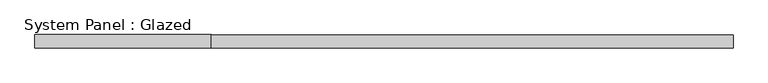
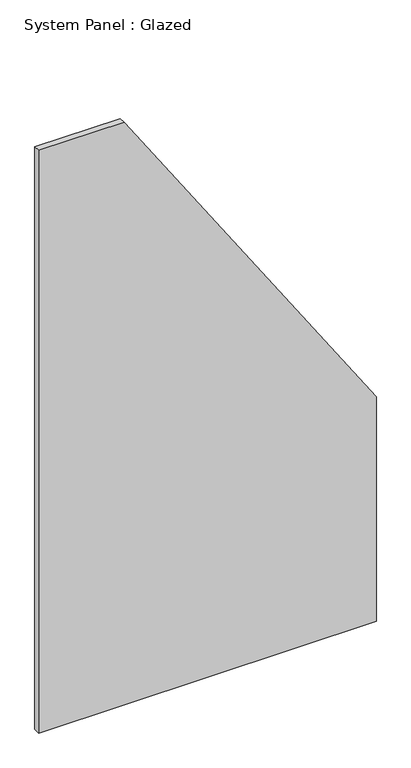
"""IFC4 building model written with IfcOpenShell, lengths in millimetres: plate geometry, System Panel : Glazed."""

from ifc_helpers import new_model, si_unit, frame, origin, place, context, project, spatial, polyline, outline, extrude, source, transform, mapped, element, save


def system_panel_glazed_e9d80b72(model_context):
    return source(origin(), model_context, "Body", "SweptSolid", [
        extrude(outline(polyline([(0.0, -658.3333333), (0.0, 658.3333333), (924.6254194, 658.3333333), (2400.0, -325.3849432), (2400.0, -658.3333333), (0.0, -658.3333333)])), frame((0.0, 24.5, 0.0), z_axis=(0.0, 1.0, 0.0), x_axis=(0.0, 0.0, 1.0)), (0.0, 0.0, 1.0), 25.0),
    ])


if __name__ == "__main__":
    model = new_model("IFC4")
    model_context = context("Model", 3, world=origin())
    ifc_project = project(units=[si_unit("LENGTHUNIT", "METRE", prefix="MILLI")], contexts=[model_context])
    site = spatial("IfcSite", under=ifc_project)
    building = spatial("IfcBuilding", under=site)
    placement = place(None, origin())
    system_panel_glazed_shape = system_panel_glazed_e9d80b72(model_context)
    element("IfcPlate", 1, ObjectType="System Panel : Glazed", at=placement, inside=building, context=model_context, shape_type="MappedRepresentation", body=[
        mapped(system_panel_glazed_shape, transform((0.0, 0.0, 0.0), x_axis=(1.0, 0.0, 0.0), y_axis=(0.0, 1.0, 0.0), z_axis=(0.0, 0.0, 1.0))),
    ])
    save(model, "model.ifc")

# Revit data of these elements
# Type "System Panel : Glazed"
#   Keynote = "H11"
#   Construction Type Id = "GSP4R"
#   Analytic Construction = "1/8 in Pilkington single glazing"
#   Visual Light Transmittance = 0.9
#   Solar Heat Gain Coefficient = 0.86
#   Heat Transfer Coefficient (U) = 6.7069 W/(m²·K)
#   Define Thermal Properties by = 1
# Element 1 (IfcPlate, "System Panel : Glazed")
#   Materials on its faces: "Glass"
# Materials
#   "Glass": class "Glass", colour RGB 0 128 192, transparency 0.9, Description = "Soda Lime Glass", Cost = 0
